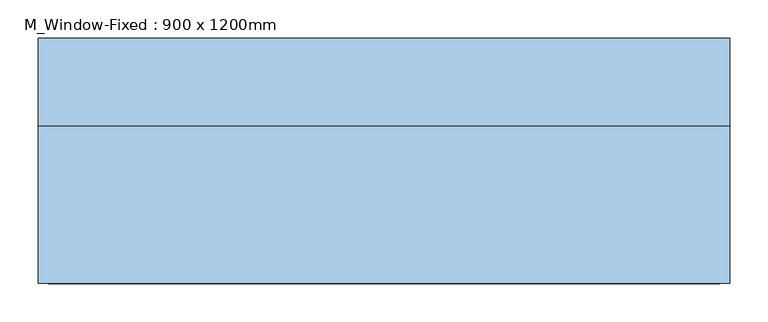
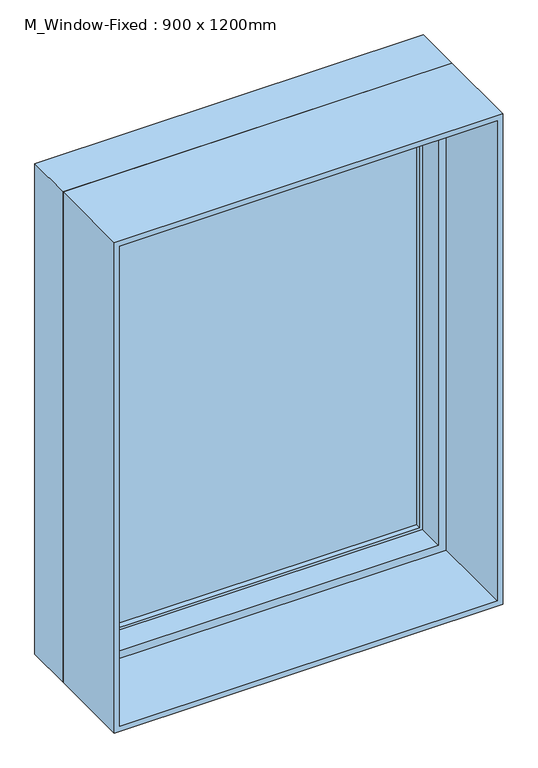
"""IFC4 building model written with IfcOpenShell, lengths in millimetres: window geometry, M_Window-Fixed : 900 x 1200mm."""

from ifc_helpers import new_model, si_unit, frame, origin, place, context, project, spatial, polyline, outline, extrude, faceted_brep, source, transform, mapped, element, save


def m_window_fixed_900_x_1200mm_d63e2c57(model_context):
    return source(origin(), model_context, "Body", "SolidModel", [
        extrude(outline(polyline([(411.9, 150.0), (411.9, 143.65), (-411.9, 143.65), (-411.9, 150.0), (411.9, 150.0)])), frame((0.0, 0.0, 938.1), z_axis=(0.0, 0.0, 1.0), x_axis=(1.0, 0.0, 0.0)), (0.0, 0.0, 1.0), 1123.8),
        extrude(outline(polyline([(-411.9, 130.95), (-411.9, 137.3), (411.9, 137.3), (411.9, 130.95), (-411.9, 130.95)])), frame((0.0, 0.0, 938.1), z_axis=(0.0, 0.0, 1.0), x_axis=(1.0, 0.0, 0.0)), (0.0, 0.0, 1.0), 1123.8),
        extrude(outline(polyline([(912.7, 437.3), (2087.3, 437.3), (2087.3, -437.3), (912.7, -437.3), (912.7, 437.3)]), holes=[polyline([(938.1, -411.9), (2061.9, -411.9), (2061.9, 411.9), (938.1, 411.9), (938.1, -411.9)])]), frame((0.0, 118.25, 0.0), z_axis=(0.0, 1.0, 0.0), x_axis=(0.0, 0.0, 1.0)), (0.0, 0.0, 1.0), 44.45),
        extrude(outline(polyline([(2100.0, -450.0), (900.0, -450.0), (900.0, 450.0), (2100.0, 450.0), (2100.0, -450.0)]), holes=[polyline([(2087.3, 437.3), (912.7, 437.3), (912.7, -437.3), (2087.3, -437.3), (2087.3, 437.3)])]), frame((0.0, -150.0, 0.0), z_axis=(0.0, 1.0, 0.0), x_axis=(0.0, 0.0, 1.0)), (0.0, 0.0, 1.0), 204.75),
        faceted_brep([(450.0, 54.75, 2100.0), (450.0, 169.05, 2100.0), (-450.0, 169.05, 2100.0), (-450.0, 54.75, 2100.0), (-450.0, 169.05, 900.0), (-450.0, 54.75, 900.0), (450.0, 169.05, 900.0), (450.0, 54.75, 900.0), (418.25, 54.75, 2068.25), (418.25, 54.75, 931.75), (-418.25, 54.75, 931.75), (-418.25, 54.75, 2068.25), (-437.3, 169.05, 2087.3), (-437.3, 169.05, 912.7), (437.3, 169.05, 912.7), (437.3, 169.05, 2087.3), (418.25, 118.25, 2068.25), (-418.25, 118.25, 2068.25), (437.3, 118.25, 2087.3), (-437.3, 118.25, 2087.3), (-418.25, 118.25, 931.75), (-437.3, 118.25, 912.7), (418.25, 118.25, 931.75), (437.3, 118.25, 912.7)], [[[0, 1, 2, 3]], [[3, 2, 4, 5]], [[5, 4, 6, 7]], [[3, 5, 7, 0], [8, 9, 10, 11]], [[7, 6, 1, 0]], [[1, 6, 4, 2], [12, 13, 14, 15]], [[16, 8, 11, 17]], [[15, 18, 19, 12]], [[17, 11, 10, 20]], [[12, 19, 21, 13]], [[20, 10, 9, 22]], [[13, 21, 23, 14]], [[22, 9, 8, 16]], [[18, 23, 21, 19], [17, 20, 22, 16]], [[14, 23, 18, 15]]]),
    ])


if __name__ == "__main__":
    model = new_model("IFC4")
    model_context = context("Model", 3, world=origin())
    ifc_project = project(units=[si_unit("LENGTHUNIT", "METRE", prefix="MILLI")], contexts=[model_context])
    site = spatial("IfcSite", under=ifc_project)
    building = spatial("IfcBuilding", under=site)
    placement = place(None, origin())
    m_window_fixed_900_x_1200mm_shape = m_window_fixed_900_x_1200mm_d63e2c57(model_context)
    element("IfcWindow", 1, ObjectType="M_Window-Fixed : 900 x 1200mm", at=placement, inside=building, context=model_context, shape_type="MappedRepresentation", body=[
        mapped(m_window_fixed_900_x_1200mm_shape, transform((0.0, 0.0, 0.0), x_axis=(1.0, 0.0, 0.0), y_axis=(0.0, 1.0, 0.0), z_axis=(0.0, 0.0, 1.0))),
    ])
    save(model, "model.ifc")

# Revit data of these elements
# Type "M_Window-Fixed : 900 x 1200mm"
#   Type Mark = "28"
#   Fire Rating = "0.5h"
#   Assembly Code = "B2020100"
#   Analytic Construction = "Double glazing - domestic"
#   Window Inset [instance default] = 0 mm
#   Wall Thickness [instance default] = 150 mm
#   Visual Light Transmittance = 0.81
#   Thermal Resistance (R) = 0.319569 (m²·K)/W
#   Solar Heat Gain Coefficient = 0.76
#   Rough Width = 915 mm
#   Rough Height = 1215 mm
#   Interior Wall Closure [instance default] = 54.75 mm
#   Height = 1200 mm
#   Heat Transfer Coefficient (U) = 3.12929 W/(m²·K)
#   Frame Extension [instance default] = 6.35 mm
#   Exterior Wall Closure [instance default] = 31.75 mm
#   Extension Jamb [instance default] = 54.75 mm
#   Default Sill Height = 900 mm
#   Width = 900 mm
#   Muntin Visibility = yes
#   Interior Trim Visibility [instance default] = yes
#   Exterior Trim Visibility [instance default] = yes
#   Extension Jamb Visibility [instance default] = yes
#   Muntin Pattern = M_Muntin Pattern_2x2 : M_Muntin Pattern_2x2
#   Interior Trim Material = Wood - Stained
#   Interior Trim = M_Trim-Window-Interior-Flat : Picture Frame
#   Interior Frame Material = Wood - Stained
#   Glass Panel Material = Glass
#   Exterior Trim Material = Clad - White
#   Exterior Trim = M_Trim-Window-Exterior-Flat : with Sill
#   Exterior Frame Material = Clad - White
#   Wall Closure = (empty or 0)
# Element 1 (IfcWindow, "M_Window-Fixed : 900 x 1200mm")
#   Wall Thickness = 300 mm
#   Extension Jamb = 204.75 mm
#   Materials on its faces: "Wood - Stained", "Glass", "Clad - White"
# Materials
#   "Wood - Stained": class "Wood", colour RGB 227 170 128, transparency 0, Cost = 0
#   "Glass": class "Glass", colour RGB 0 0 255, transparency 0.75
#   "Clad - White": class "Wood", colour RGB 242 242 238, transparency 0, Cost = 0
